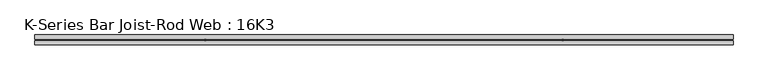
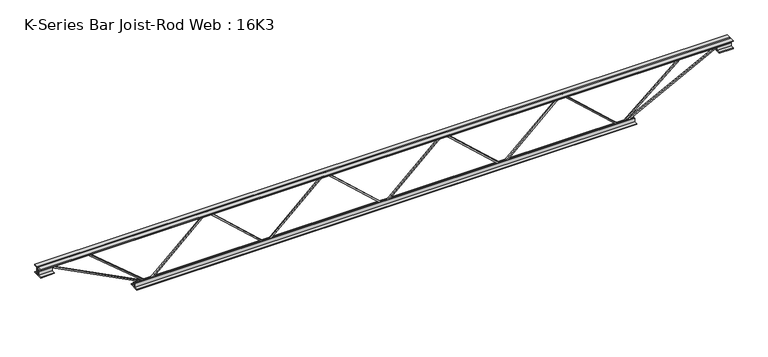
"""IFC4 building model written with IfcOpenShell, lengths in millimetres: beam geometry, K-Series Bar Joist-Rod Web : 16K3."""

from ifc_helpers import new_model, si_unit, frame, origin, place, context, project, spatial, polyline, outline, extrude, source, transform, mapped, element, save


def k_series_bar_joist_rod_web_16k3_40919eac(model_context):
    return source(origin(), model_context, "Body", "SweptSolid", [
        extrude(outline(polyline([(-192.0875, 0.0), (-201.6125, 0.0), (-201.6125, 5.0233558), (192.0875, 435.8311683), (192.0875, 438.4844567), (-201.6125, 869.2922692), (-201.6125, 874.315625), (-192.0875, 874.315625), (-192.0875, 872.9889808), (201.6125, 442.1811683), (201.6125, 432.1344567), (-192.0875, 1.3266442), (-192.0875, 0.0)])), frame((0.0, -4.7625, 0.0), z_axis=(0.0, 1.0, 0.0), x_axis=(0.0, 0.0, 1.0)), (0.0, 0.0, 1.0), 9.525),
        extrude(outline(polyline([(-192.0875, -874.315625), (-201.6125, -874.315625), (-201.6125, -869.2922692), (192.0875, -438.4844567), (192.0875, -435.8311683), (-201.6125, -5.0233558), (-201.6125, 0.0), (-192.0875, 0.0), (-192.0875, -1.3266442), (201.6125, -432.1344567), (201.6125, -442.1811683), (-192.0875, -872.9889808), (-192.0875, -874.315625)])), frame((0.0, -4.7625, 0.0), z_axis=(0.0, 1.0, 0.0), x_axis=(0.0, 0.0, 1.0)), (0.0, 0.0, 1.0), 9.525),
        extrude(outline(polyline([(-192.0875, 874.315625), (-201.6125, 874.315625), (-201.6125, 879.3389808), (192.0875, 1310.1467933), (192.0875, 1312.8000817), (-201.6125, 1743.6078942), (-201.6125, 1748.63125), (-192.0875, 1748.63125), (-192.0875, 1747.3046058), (201.6125, 1316.4967933), (201.6125, 1306.4500817), (-192.0875, 875.6422692), (-192.0875, 874.315625)])), frame((0.0, -4.7625, 0.0), z_axis=(0.0, 1.0, 0.0), x_axis=(0.0, 0.0, 1.0)), (0.0, 0.0, 1.0), 9.525),
        extrude(outline(polyline([(-192.0875, -1748.63125), (-201.6125, -1748.63125), (-201.6125, -1743.6078942), (192.0875, -1312.8000817), (192.0875, -1310.1467933), (-201.6125, -879.3389808), (-201.6125, -874.315625), (-192.0875, -874.315625), (-192.0875, -875.6422692), (201.6125, -1306.4500817), (201.6125, -1316.4967933), (-192.0875, -1747.3046058), (-192.0875, -1748.63125)])), frame((0.0, -4.7625, 0.0), z_axis=(0.0, 1.0, 0.0), x_axis=(0.0, 0.0, 1.0)), (0.0, 0.0, 1.0), 9.525),
        extrude(outline(polyline([(4.7625, 203.2), (36.5125, 203.2), (36.5125, 196.85), (11.1125, 196.85), (11.1125, 171.45), (4.7625, 171.45), (4.7625, 203.2)])), frame((-2561.43125, 0.0, 0.0), z_axis=(1.0, 0.0, 0.0), x_axis=(0.0, 1.0, 0.0)), (0.0, 0.0, 1.0), 5122.8625),
        extrude(outline(polyline([(-4.7625, 203.2), (-4.7625, 171.45), (-11.1125, 171.45), (-11.1125, 196.85), (-36.5125, 196.85), (-36.5125, 203.2), (-4.7625, 203.2)])), frame((-2561.43125, 0.0, 0.0), z_axis=(1.0, 0.0, 0.0), x_axis=(0.0, 1.0, 0.0)), (0.0, 0.0, 1.0), 5122.8625),
        extrude(outline(polyline([(-4.7625, 139.7), (-36.5125, 139.7), (-36.5125, 146.05), (-11.1125, 146.05), (-11.1125, 171.45), (-4.7625, 171.45), (-4.7625, 139.7)])), frame((-2561.43125, 0.0, 0.0), z_axis=(1.0, 0.0, 0.0), x_axis=(0.0, 1.0, 0.0)), (0.0, 0.0, 1.0), 101.6),
        extrude(outline(polyline([(36.5125, 139.7), (4.7625, 139.7), (4.7625, 171.45), (11.1125, 171.45), (11.1125, 146.05), (36.5125, 146.05), (36.5125, 139.7)])), frame((-2561.43125, 0.0, 0.0), z_axis=(1.0, 0.0, 0.0), x_axis=(0.0, 1.0, 0.0)), (0.0, 0.0, 1.0), 101.6),
        extrude(outline(polyline([(4.7625, 139.7), (4.7625, 171.45), (11.1125, 171.45), (11.1125, 146.05), (36.5125, 146.05), (36.5125, 139.7), (4.7625, 139.7)])), frame((2459.83125, 0.0, 0.0), z_axis=(1.0, 0.0, 0.0), x_axis=(0.0, 1.0, 0.0)), (0.0, 0.0, 1.0), 101.6),
        extrude(outline(polyline([(-4.7625, 139.7), (-36.5125, 139.7), (-36.5125, 146.05), (-11.1125, 146.05), (-11.1125, 171.45), (-4.7625, 171.45), (-4.7625, 139.7)])), frame((2459.83125, 0.0, 0.0), z_axis=(1.0, 0.0, 0.0), x_axis=(0.0, 1.0, 0.0)), (0.0, 0.0, 1.0), 101.6),
        extrude(outline(polyline([(4.7625, -203.2), (4.7625, -171.45), (11.1125, -171.45), (11.1125, -196.85), (36.5125, -196.85), (36.5125, -203.2), (4.7625, -203.2)])), frame((-1850.23125, 0.0, 0.0), z_axis=(1.0, 0.0, 0.0), x_axis=(0.0, 1.0, 0.0)), (0.0, 0.0, 1.0), 3700.4625),
        extrude(outline(polyline([(-4.7625, -203.2), (-36.5125, -203.2), (-36.5125, -196.85), (-11.1125, -196.85), (-11.1125, -171.45), (-4.7625, -171.45), (-4.7625, -203.2)])), frame((-1850.23125, 0.0, 0.0), z_axis=(1.0, 0.0, 0.0), x_axis=(0.0, 1.0, 0.0)), (0.0, 0.0, 1.0), 3700.4625),
        extrude(outline(polyline([(0.0, -9.525), (0.0, 0.0), (800.9059433, 0.0), (800.9059433, -9.525), (0.0, -9.525)])), frame((-2462.0213059, 4.7625, 167.2209266), z_axis=(0.459854247661137, 0.0, 0.8879944092774513), x_axis=(0.8879944092774513, 0.0, -0.459854247661137)), (0.0, 0.0, 1.0), 9.525),
        extrude(outline(polyline([(0.0, -9.525), (0.0, 0.0), (571.6221156, 0.0), (571.6221156, -9.525), (0.0, -9.525)])), frame((-2188.8575735, 4.7625, 167.8077965), z_axis=(0.644306771827224, 0.0, 0.7647671435002825), x_axis=(0.7647671435002825, 0.0, -0.644306771827224)), (0.0, 0.0, 1.0), 9.525),
        extrude(outline(polyline([(0.0, -9.525), (0.0, 0.0), (800.9059433, 0.0), (800.9059433, -9.525), (0.0, -9.525)])), frame((2462.0213059, -4.7625, 167.2209266), z_axis=(-0.4598542476611237, 0.0, 0.8879944092774583), x_axis=(-0.8879944092774583, 0.0, -0.4598542476611237)), (0.0, 0.0, 1.0), 9.525),
        extrude(outline(polyline([(0.0, -9.525), (0.0, 0.0), (571.6221156, 0.0), (571.6221156, -9.525), (0.0, -9.525)])), frame((2188.8575735, -4.7625, 167.8077965), z_axis=(-0.6443067718272195, 0.0, 0.7647671435002863), x_axis=(-0.7647671435002863, 0.0, -0.6443067718272195)), (0.0, 0.0, 1.0), 9.525),
    ])


if __name__ == "__main__":
    model = new_model("IFC4")
    model_context = context("Model", 3, world=origin())
    ifc_project = project(units=[si_unit("LENGTHUNIT", "METRE", prefix="MILLI")], contexts=[model_context])
    site = spatial("IfcSite", under=ifc_project)
    building = spatial("IfcBuilding", under=site)
    placement = place(None, origin())
    k_series_bar_joist_rod_web_16k3_shape = k_series_bar_joist_rod_web_16k3_40919eac(model_context)
    element("IfcBeam", 1, ObjectType="K-Series Bar Joist-Rod Web : 16K3", at=placement, inside=building, context=model_context, shape_type="MappedRepresentation", body=[
        mapped(k_series_bar_joist_rod_web_16k3_shape, transform((0.0, 0.0, 0.0), x_axis=(1.0, 0.0, 0.0), y_axis=(0.0, 1.0, 0.0), z_axis=(0.0, 0.0, 1.0))),
    ])
    save(model, "model.ifc")

# Revit data of these elements
# Type "K-Series Bar Joist-Rod Web : 16K3"
#   Assembly Code = "B1010350"
#   Wt = 6.3
#   Web Thickness = 0' - 0 3/8"
#   Start Offset [instance default] = 0' - 0"
#   Start Extension [instance default] = 0' - 0"
#   Seat Length = 0' - 4"
#   Seat Depth = 0' - 2 1/2"
#   PanelArrayLength [instance default] = 18' - 8"
#   Panel [instance default] = 2' - 8"
#   End Offset [instance default] = 0' - 0"
#   End Extension [instance default] = 0' - 0"
#   End Panel = 2' - 8"
#   Cord Leg = 0' - 1 1/4"
#   Chord Thickness = 0' - 0 1/4"
#   Length [instance default] = 24' - 0"
#   Depth = 1' - 4"
#   PanelArrayNum [instance default] = 7
#   Structural Material = none
# Element 1 (IfcBeam, "K-Series Bar Joist-Rod Web : 16K3")
#   PanelArrayLength = 11' - 5 11/16"
#   Panel = 2' - 10 27/64"
#   PanelArrayNum = 4
